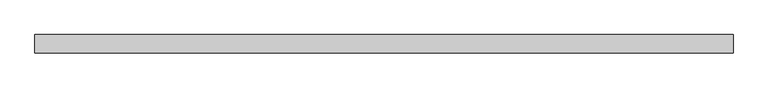
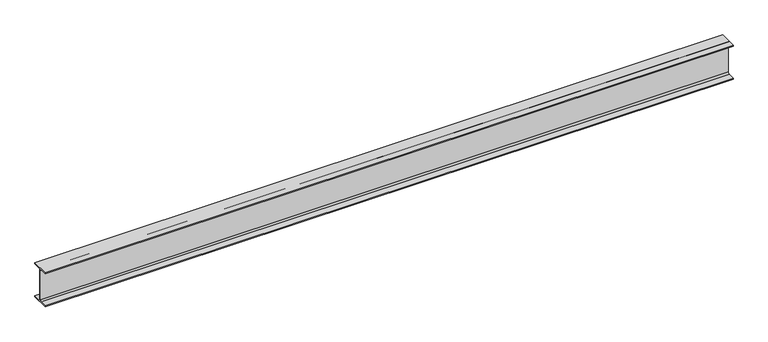
"""IFC4 building model written with IfcOpenShell, lengths in millimetres: beam geometry, Steel Framing_H_KS : H_SB_AR_S02_H-300x150x6.5x9_SRB3."""

from ifc_helpers import new_model, si_unit, point, frame, frame_2d, origin, place, context, project, spatial, polyline, circle_curve, trimmed, segment, composite_curve, outline, extrude, source, transform, mapped, element, save


def beam_b3b7c95e(model_context):
    return source(origin(), model_context, "Body", "SweptSolid", [
        extrude(outline(composite_curve([segment(polyline([(75.0, -141.0), (75.0, -150.0), (-75.0, -150.0), (-75.0, -141.0), (-16.25, -141.0)]), True, "CONTINUOUS"), segment(trimmed(circle_curve(frame_2d((-16.25, -128.0)), 13.0), [point((-16.25, -141.0))], [point((-3.25, -128.0))], True, "CARTESIAN"), True, "CONTINUOUS"), segment(polyline([(-3.25, -128.0), (-3.25, 128.0)]), True, "CONTINUOUS"), segment(trimmed(circle_curve(frame_2d((-16.25, 128.0)), 13.0), [point((-3.25, 128.0))], [point((-16.25, 141.0))], True, "CARTESIAN"), True, "CONTINUOUS"), segment(polyline([(-16.25, 141.0), (-75.0, 141.0), (-75.0, 150.0), (75.0, 150.0), (75.0, 141.0), (16.25, 141.0)]), True, "CONTINUOUS"), segment(trimmed(circle_curve(frame_2d((16.25, 128.0)), 13.0), [point((16.25, 141.0))], [point((3.25, 128.0))], True, "CARTESIAN"), True, "CONTINUOUS"), segment(polyline([(3.25, 128.0), (3.25, -128.0)]), True, "CONTINUOUS"), segment(trimmed(circle_curve(frame_2d((16.25, -128.0)), 13.0), [point((3.25, -128.0))], [point((16.25, -141.0))], True, "CARTESIAN"), True, "CONTINUOUS"), segment(polyline([(16.25, -141.0), (75.0, -141.0)]), True, "CONTINUOUS")], self_intersect=False)), frame((-2912.3, 0.0, 0.0), z_axis=(1.0, 0.0, 0.0), x_axis=(0.0, 1.0, 0.0)), (0.0, 0.0, 1.0), 5749.6),
    ])


if __name__ == "__main__":
    model = new_model("IFC4")
    model_context = context("Model", 3, world=origin())
    ifc_project = project(units=[si_unit("LENGTHUNIT", "METRE", prefix="MILLI")], contexts=[model_context])
    site = spatial("IfcSite", under=ifc_project)
    building = spatial("IfcBuilding", under=site)
    placement = place(None, origin())
    beam_shape = beam_b3b7c95e(model_context)
    element("IfcBeam", 1, ObjectType="Steel Framing_H_KS : H_SB_AR_S02_H-300x150x6.5x9_SRB3", at=placement, inside=building, context=model_context, shape_type="MappedRepresentation", body=[
        mapped(beam_shape, transform((0.0, 0.0, 0.0), x_axis=(1.0, 0.0, 0.0), y_axis=(0.0, 1.0, 0.0), z_axis=(0.0, 0.0, 1.0))),
    ])
    save(model, "model.ifc")

# Revit data of these elements
# Type "Steel Framing_H_KS : H_SB_AR_S02_H-300x150x6.5x9_SRB3"
#   Type Comments = "MAIN"
#   Type Mark = "SRB3"
#   H_SectionID = "H-300x150x6.5x9"
#   H_Ratio for Additional Steel Plate = 0.2
#   Width = 15.0 cm
#   Web Thickness = 0.65 cm
#   Web Fillet = 1.3 cm
#   Warping Constant = 107000.0 cm⁶
#   Torsional Moment of Inertia = 9.9539 cm⁴
#   Section Area = 46.78 cm²
#   Plastic Modulus weak axis = 105.0 cm³
#   Plastic Modulus strong axis = 542.0 cm³
#   Perimeter = 1.17 m²/m
#   Nominal Weight = 36.70 kgf/m
#   Moment of Inertia weak axis = 508.00 cm⁴
#   Moment of Inertia strong axis = 7210.00 cm⁴
#   Height = 30.0 cm
#   Flange Thickness = 0.9 cm
#   Elastic Modulus weak axis = 67.7 cm³
#   Elastic Modulus strong axis = 481.0 cm³
#   Centroid Vertical = 15.0 cm
#   Centroid Horizontal = 7.5 cm
#   Bolt Spacing = 8.89 cm
#   Length [instance default] = 1500 mm
#   Structural Material [instance default] = Steel, 45-345
#   Section Name Key = ""
#   Assembly Code = ""
# Element 1 (IfcBeam, "Steel Framing_H_KS : H_SB_AR_S02_H-300x150x6.5x9_SRB3")
#   Materials on its faces: "Steel, 45-345"
# Materials
#   "Steel, 45-345": class "Metal", colour RGB 189 187 185, transparency 0, Description = "Steel 345 MPa", Cost = 0
